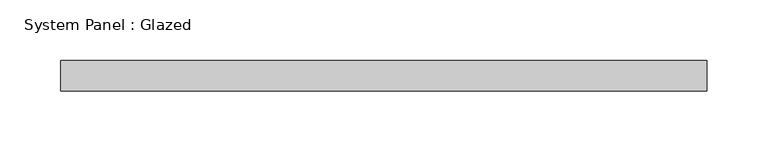
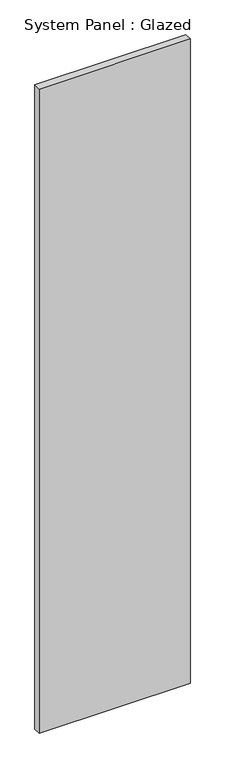
"""IFC4 building model written with IfcOpenShell, lengths in millimetres: plate geometry, System Panel : Glazed."""

from ifc_helpers import new_model, si_unit, origin, origin_with_axes, place, context, project, spatial, polyline, outline, extrude, source, transform, mapped, element, save


def system_panel_glazed_8581e904(model_context):
    return source(origin(), model_context, "Body", "SweptSolid", [
        extrude(outline(polyline([(266.25, 24.5), (-266.25, 24.5), (-266.25, 49.5), (266.25, 49.5), (266.25, 24.5)])), origin_with_axes(), (0.0, 0.0, 1.0), 2400.0),
    ])


if __name__ == "__main__":
    model = new_model("IFC4")
    model_context = context("Model", 3, world=origin())
    ifc_project = project(units=[si_unit("LENGTHUNIT", "METRE", prefix="MILLI")], contexts=[model_context])
    site = spatial("IfcSite", under=ifc_project)
    building = spatial("IfcBuilding", under=site)
    placement = place(None, origin())
    system_panel_glazed_shape = system_panel_glazed_8581e904(model_context)
    element("IfcPlate", 1, ObjectType="System Panel : Glazed", at=placement, inside=building, context=model_context, shape_type="MappedRepresentation", body=[
        mapped(system_panel_glazed_shape, transform((0.0, 0.0, 0.0), x_axis=(1.0, 0.0, 0.0), y_axis=(0.0, 1.0, 0.0), z_axis=(0.0, 0.0, 1.0))),
    ])
    save(model, "model.ifc")

# Revit data of these elements
# Type "System Panel : Glazed"
#   Keynote = "H11"
#   Construction Type Id = "GSP4R"
#   Analytic Construction = "1/8 in Pilkington single glazing"
#   Visual Light Transmittance = 0.9
#   Solar Heat Gain Coefficient = 0.86
#   Heat Transfer Coefficient (U) = 6.7069 W/(m²·K)
#   Define Thermal Properties by = 1
# Element 1 (IfcPlate, "System Panel : Glazed")
#   Materials on its faces: "Glass"
# Materials
#   "Glass": class "Glass", colour RGB 0 128 192, transparency 0.9, Description = "Soda Lime Glass", Cost = 0
